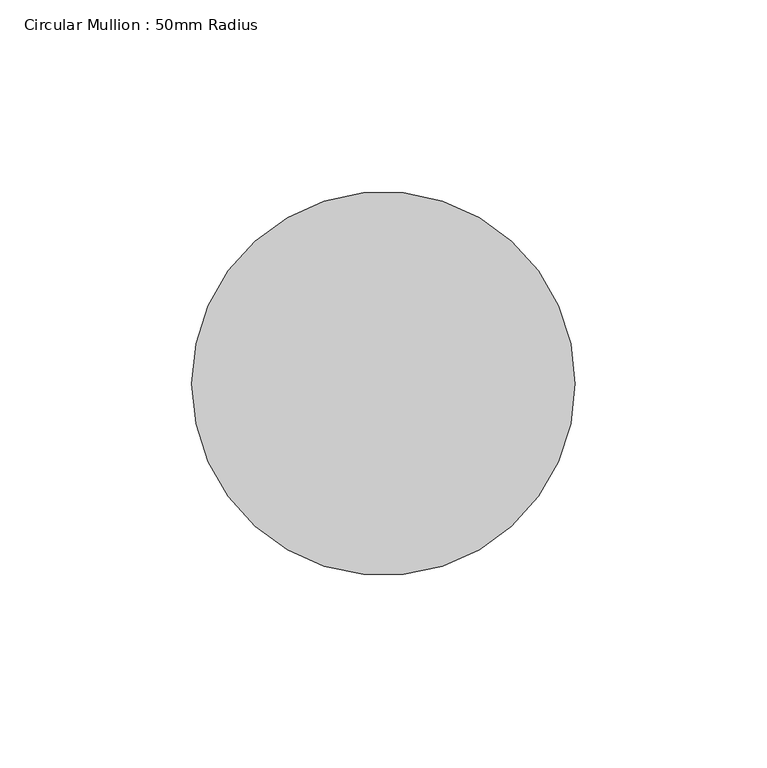
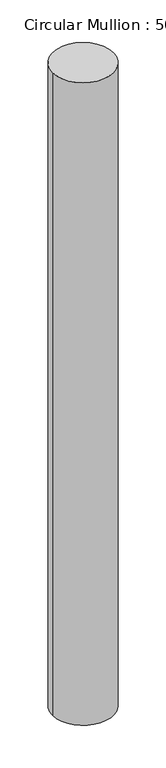
"""IFC4 building model written with IfcOpenShell, lengths in millimetres: member geometry, Circular Mullion : 50mm Radius."""

from ifc_helpers import new_model, si_unit, point, frame, origin, origin_2d, place, context, project, spatial, circle_curve, trimmed, segment, composite_curve, outline, extrude, source, transform, mapped, element, save


def circular_mullion_50mm_radius_4c7d2050(model_context):
    return source(origin(), model_context, "Body", "SweptSolid", [
        extrude(outline(composite_curve([segment(trimmed(circle_curve(origin_2d(), 50.0), [point((50.0, 0.0))], [point((-50.0, 0.0))], False, "CARTESIAN"), True, "CONTINUOUS"), segment(trimmed(circle_curve(origin_2d(), 50.0), [point((-50.0, 0.0))], [point((50.0, 0.0))], False, "CARTESIAN"), True, "CONTINUOUS")], self_intersect=False)), frame((0.0, 0.0, -1115.9805772), z_axis=(0.0, 0.0, 1.0), x_axis=(1.0, 0.0, 0.0)), (0.0, 0.0, 1.0), 1115.9805772),
    ])


if __name__ == "__main__":
    model = new_model("IFC4")
    model_context = context("Model", 3, world=origin())
    ifc_project = project(units=[si_unit("LENGTHUNIT", "METRE", prefix="MILLI")], contexts=[model_context])
    site = spatial("IfcSite", under=ifc_project)
    building = spatial("IfcBuilding", under=site)
    placement = place(None, origin())
    circular_mullion_50mm_radius_shape = circular_mullion_50mm_radius_4c7d2050(model_context)
    element("IfcMember", 1, ObjectType="Circular Mullion : 50mm Radius", at=placement, inside=building, context=model_context, shape_type="MappedRepresentation", body=[
        mapped(circular_mullion_50mm_radius_shape, transform((0.0, 0.0, 0.0), x_axis=(1.0, 0.0, 0.0), y_axis=(0.0, 1.0, 0.0), z_axis=(0.0, 0.0, 1.0))),
    ])
    save(model, "model.ifc")

# Revit data of these elements
# Type "Circular Mullion : 50mm Radius"
#   built-in parameter 1007350 = 0.164042 (stored number, unit not read)
# Element 1 (IfcMember, "Circular Mullion : 50mm Radius")
#   Materials on its faces: "Aluminium"
# Materials
#   "Aluminium": class "Metal", colour RGB 247 247 247, transparency 0, Description = "Aluminium 6061", Cost = 0
